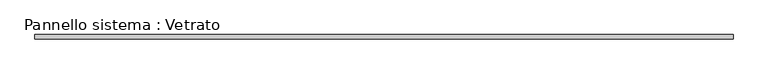
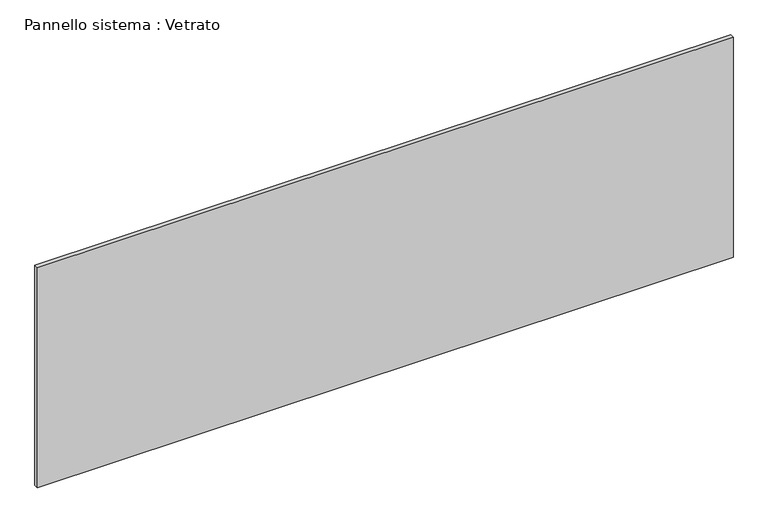
"""IFC4 building model written with IfcOpenShell, lengths in millimetres: plate geometry, Pannello sistema : Vetrato."""

from ifc_helpers import new_model, si_unit, origin, origin_with_axes, place, context, project, spatial, polyline, outline, extrude, source, transform, mapped, element, save


def pannello_sistema_vetrato_f11d9790(model_context):
    return source(origin(), model_context, "Body", "SweptSolid", [
        extrude(outline(polyline([(2460.0, -15.0), (-2460.0, -15.0), (-2460.0, 15.0), (2460.0, 15.0), (2460.0, -15.0)])), origin_with_axes(), (0.0, 0.0, 1.0), 1645.0),
    ])


if __name__ == "__main__":
    model = new_model("IFC4")
    model_context = context("Model", 3, world=origin())
    ifc_project = project(units=[si_unit("LENGTHUNIT", "METRE", prefix="MILLI")], contexts=[model_context])
    site = spatial("IfcSite", under=ifc_project)
    building = spatial("IfcBuilding", under=site)
    placement = place(None, origin())
    pannello_sistema_vetrato_shape = pannello_sistema_vetrato_f11d9790(model_context)
    element("IfcPlate", 1, ObjectType="Pannello sistema : Vetrato", at=placement, inside=building, context=model_context, shape_type="MappedRepresentation", body=[
        mapped(pannello_sistema_vetrato_shape, transform((0.0, 0.0, 0.0), x_axis=(1.0, 0.0, 0.0), y_axis=(0.0, 1.0, 0.0), z_axis=(0.0, 0.0, 1.0))),
    ])
    save(model, "model.ifc")

# Revit data of these elements
# Type "Pannello sistema : Vetrato"
#   Construction Type Id = "GSP4R"
#   Analytic Construction = "Vetrata singola Pilkington 1/8 in"
#   Visual Light Transmittance = 0.9
#   Solar Heat Gain Coefficient = 0.86
#   Heat Transfer Coefficient (U) = 6.7069 W/(m²·K)
# Element 1 (IfcPlate, "Pannello sistema : Vetrato")
#   Materials on its faces: "Default - Vetro"
# Materials
#   "Default - Vetro": class "Vetro", colour RGB 208 208 208, transparency 0.7, Cost = 0
